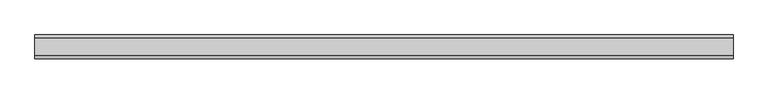
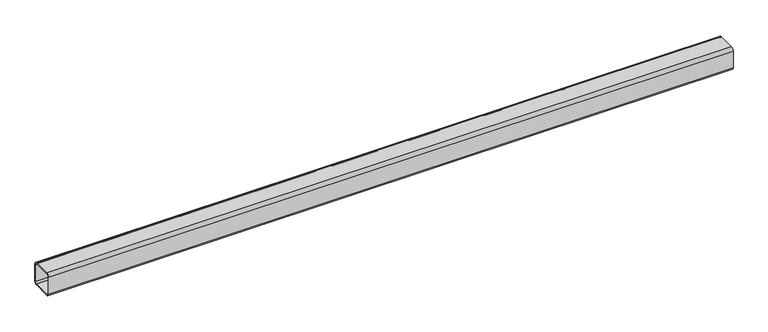
"""IFC4 building model written with IfcOpenShell, lengths in millimetres: beam geometry, Гнутый прямоугольный профиль (Трубы 30245-94) Балки : гнутый прямоуг. проф. 100x6."""

from ifc_helpers import new_model, si_unit, point, frame, frame_2d, origin, place, context, project, spatial, polyline, circle_curve, trimmed, segment, composite_curve, outline, extrude, source, transform, mapped, element, save


def beam_f1ee62be(model_context):
    return source(origin(), model_context, "Body", "SweptSolid", [
        extrude(outline(composite_curve([segment(polyline([(-38.0, 50.0), (38.0, 50.0)]), True, "CONTINUOUS"), segment(trimmed(circle_curve(frame_2d((38.0, 38.0)), 12.0), [point((38.0, 50.0))], [point((50.0, 38.0))], False, "CARTESIAN"), True, "CONTINUOUS"), segment(polyline([(50.0, 38.0), (50.0, -38.0)]), True, "CONTINUOUS"), segment(trimmed(circle_curve(frame_2d((38.0, -38.0)), 12.0), [point((50.0, -38.0))], [point((38.0, -50.0))], False, "CARTESIAN"), True, "CONTINUOUS"), segment(polyline([(38.0, -50.0), (-38.0, -50.0)]), True, "CONTINUOUS"), segment(trimmed(circle_curve(frame_2d((-38.0, -38.0)), 12.0), [point((-38.0, -50.0))], [point((-50.0, -38.0))], False, "CARTESIAN"), True, "CONTINUOUS"), segment(polyline([(-50.0, -38.0), (-50.0, 38.0)]), True, "CONTINUOUS"), segment(trimmed(circle_curve(frame_2d((-38.0, 38.0)), 12.0), [point((-50.0, 38.0))], [point((-38.0, 50.0))], False, "CARTESIAN"), True, "CONTINUOUS")], self_intersect=False), holes=[composite_curve([segment(trimmed(circle_curve(frame_2d((-38.0, 38.0)), 6.0), [point((-38.0, 44.0))], [point((-44.0, 38.0))], True, "CARTESIAN"), True, "CONTINUOUS"), segment(polyline([(-44.0, 38.0), (-44.0, -38.0)]), True, "CONTINUOUS"), segment(trimmed(circle_curve(frame_2d((-38.0, -38.0)), 6.0), [point((-44.0, -38.0))], [point((-38.0, -44.0))], True, "CARTESIAN"), True, "CONTINUOUS"), segment(polyline([(-38.0, -44.0), (38.0, -44.0)]), True, "CONTINUOUS"), segment(trimmed(circle_curve(frame_2d((38.0, -38.0)), 6.0), [point((38.0, -44.0))], [point((44.0, -38.0))], True, "CARTESIAN"), True, "CONTINUOUS"), segment(polyline([(44.0, -38.0), (44.0, 38.0)]), True, "CONTINUOUS"), segment(trimmed(circle_curve(frame_2d((38.0, 38.0)), 6.0), [point((44.0, 38.0))], [point((38.0, 44.0))], True, "CARTESIAN"), True, "CONTINUOUS"), segment(polyline([(38.0, 44.0), (-38.0, 44.0)]), True, "CONTINUOUS")], self_intersect=False)]), frame((-1460.5, 0.0, 0.0), z_axis=(1.0, 0.0, 0.0), x_axis=(0.0, 1.0, 0.0)), (0.0, 0.0, 1.0), 2921.0),
    ])


if __name__ == "__main__":
    model = new_model("IFC4")
    model_context = context("Model", 3, world=origin())
    ifc_project = project(units=[si_unit("LENGTHUNIT", "METRE", prefix="MILLI")], contexts=[model_context])
    site = spatial("IfcSite", under=ifc_project)
    building = spatial("IfcBuilding", under=site)
    placement = place(None, origin())
    beam_shape = beam_f1ee62be(model_context)
    element("IfcBeam", 1, ObjectType="Гнутый прямоугольный профиль (Трубы 30245-94) Балки : гнутый прямоуг. проф. 100x6", at=placement, inside=building, context=model_context, shape_type="MappedRepresentation", body=[
        mapped(beam_shape, transform((0.0, 0.0, 0.0), x_axis=(1.0, 0.0, 0.0), y_axis=(0.0, 1.0, 0.0), z_axis=(0.0, 0.0, 1.0))),
    ])
    save(model, "model.ifc")

# Revit data of these elements
# Type "Гнутый прямоугольный профиль (Трубы 30245-94) Балки : гнутый прямоуг. проф. 100x6"
#   ri = 12 mm
#   ra = 6 mm
#   W = 0.173578
#   Vz = 50 mm
#   Vy = 50 mm
#   Vpz = 50 mm
#   Vpy = 50 mm
#   Length [instance default] = 1500 mm
#   bf = 100 mm
#   d = 100 mm
#   tf = 6 mm
#   tw = 6 mm
#   A = 0.00226 m²
#   Structural Material [instance default] = Металл - Сталь - 345 МПa
#   Assembly Code = ""
# Element 1 (IfcBeam, "Гнутый прямоугольный профиль (Трубы 30245-94) Балки : гнутый прямоуг. проф. 100x6")
#   Structural Material = C235
#   Materials on its faces: "C235"
# Materials
#   "Металл - Сталь - 345 МПa": class "Металл", colour RGB 247 247 247, transparency 0
#   "C235": class "Не назначено", colour RGB 0 0 0, transparency 0
